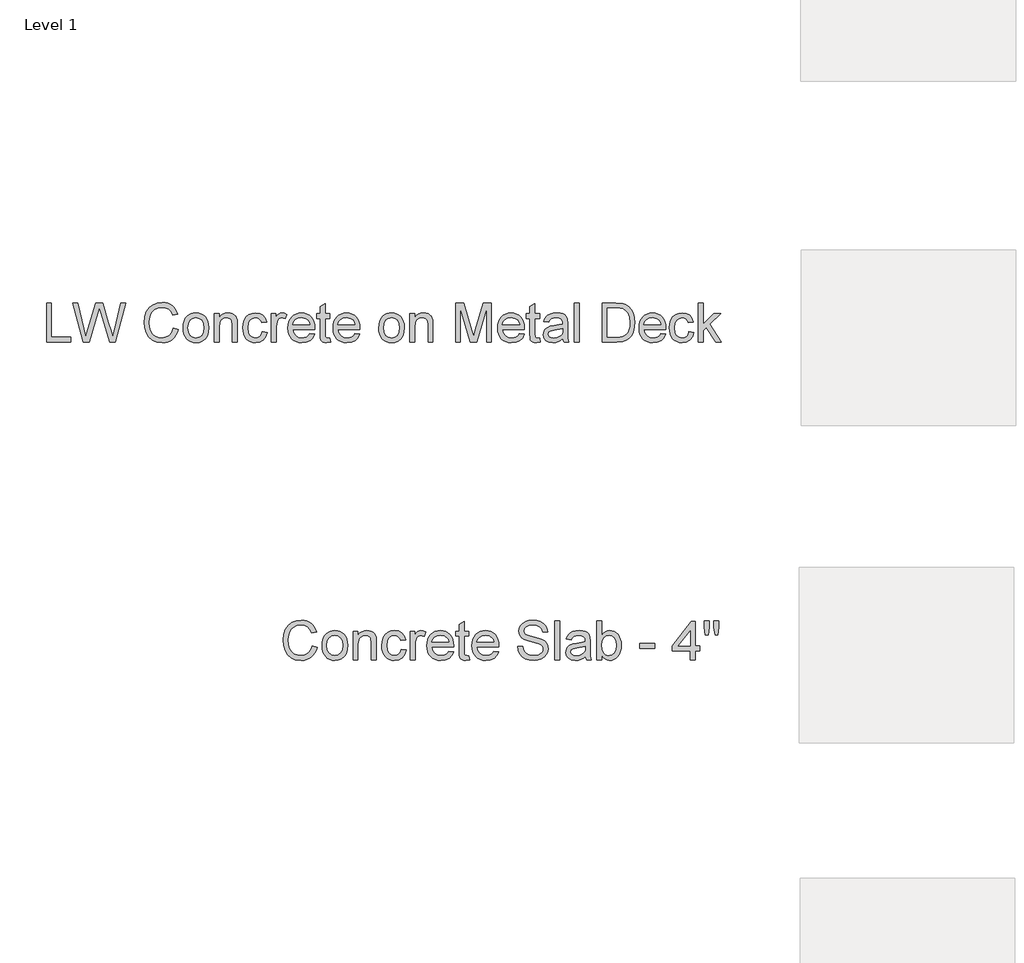
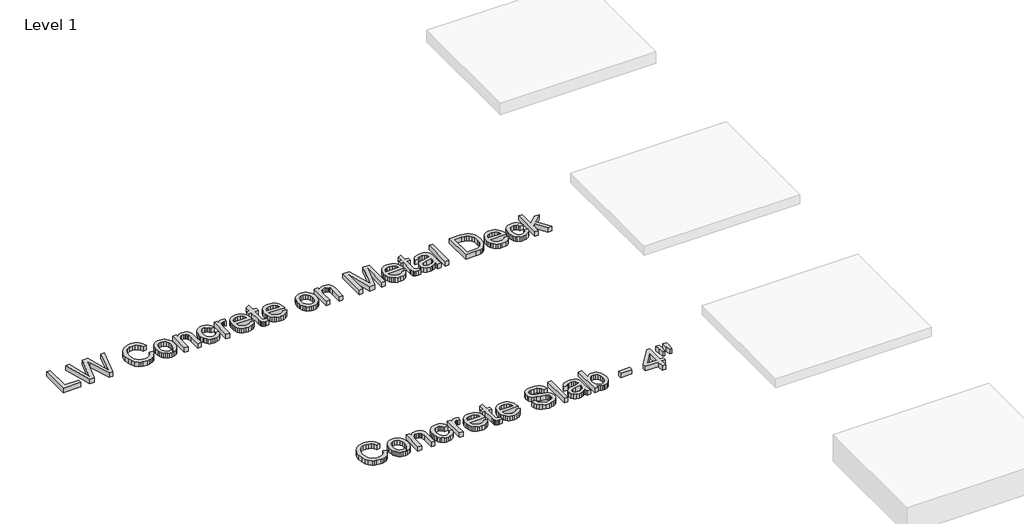
# One storey, part 13 of 42: 2 proxies.
"""IFC4 building model written with IfcOpenShell, lengths in millimetres."""

from ifc_helpers import new_model, si_unit, origin, origin_with_axes, place, context, project, spatial, polyline, outline, extrude, element, save

model = new_model("IFC4")

# Units and contexts
model_context = context("Model", 3, world=origin())
ifc_project = project(units=[si_unit("LENGTHUNIT", "METRE", prefix="MILLI")], contexts=[model_context])

# Site, building, storey
site = spatial("IfcSite", under=ifc_project)
building = spatial("IfcBuilding", under=site)
storey = spatial("IfcBuildingStorey", under=building, Name="Level 1", Elevation=0.0)

# Proxies
placement = place(None, origin())
element("IfcBuildingElementProxy", 1, Name="8\" Arial", ObjectType="8\" Arial", at=placement, inside=storey, context=model_context, shape_type="SweptSolid", body=[
    extrude(outline(polyline([(17896.3774302, -8659.233143), (17896.3774302, -8354.6660489), (17934.448317, -8354.6660489), (17934.448317, -8621.1622562), (18086.731864, -8621.1622562), (18086.731864, -8659.233143), (17896.3774302, -8659.233143)])), origin_with_axes(), (0.0, 0.0, 1.0), 50.8),
    extrude(outline(polyline([(18184.0654397, -8659.233143), (18101.0084465, -8354.6660489), (18140.2690485, -8354.6660489), (18188.4525146, -8554.8356332), (18203.3239547, -8616.626467), (18219.2363956, -8561.9739245), (18279.6144426, -8354.6660489), (18336.2002723, -8354.6660489), (18380.0710208, -8504.9419515), (18398.8648032, -8560.7098521), (18412.7138319, -8616.626467), (18427.1391288, -8556.620206), (18475.7687381, -8354.6660489), (18515.02934, -8354.6660489), (18431.8979897, -8659.233143), (18391.2246009, -8659.233143), (18318.2058298, -8424.2643888), (18308.0188933, -8391.4728633), (18296.5678844, -8430.9565368), (18230.0181897, -8659.233143), (18184.0654397, -8659.233143)])), origin_with_axes(), (0.0, 0.0, 1.0), 50.8),
    extrude(outline(polyline([(18886.2204859, -8550.9690588), (18924.2913727, -8560.7842093), (18916.7580588, -8584.4600067), (18906.724484, -8605.1475741), (18894.1906484, -8622.8469116), (18879.1565519, -8637.558019), (18861.9614492, -8649.1228874), (18842.9445951, -8657.3835076), (18822.1059896, -8662.3398798), (18799.4456327, -8663.9920038), (18755.2867501, -8658.9914821), (18736.6161218, -8652.7408299), (18720.2180354, -8643.9899168), (18693.3379073, -8619.5078085), (18673.7447849, -8586.0656575), (18661.7825703, -8546.7492876), (18657.7951654, -8504.6445227), (18662.3030707, -8460.2346846), (18675.8267865, -8421.8849584), (18697.6599196, -8390.8129431), (18727.0960764, -8368.236238), (18762.0067822, -8354.4894506), (18800.2635619, -8349.9071881), (18822.0386034, -8351.3896848), (18842.0058355, -8355.8371748), (18860.1652581, -8363.2496583), (18876.5168712, -8373.6271351), (18890.7911301, -8386.6954131), (18902.7184898, -8402.1803002), (18919.5325118, -8440.3999013), (18881.4616251, -8449.4714798), (18868.263222, -8421.70836), (18850.2316008, -8402.663622), (18827.14369, -8391.6494616), (18798.7764179, -8387.9780748), (18766.0778389, -8392.0491316), (18739.2163001, -8404.2623018), (18718.8331325, -8423.3349238), (18705.5696668, -8447.9843358), (18698.2919558, -8475.8496968), (18695.8660521, -8504.5701655), (18698.738099, -8539.7411215), (18707.3542396, -8570.1532165), (18722.0397868, -8594.6446195), (18743.1200532, -8612.0534991), (18768.3922068, -8622.4542126), (18795.6534155, -8625.9211171), (18827.4318241, -8621.1994348), (18853.9122822, -8607.0343881), (18873.9050746, -8583.5746913), (18886.2204859, -8550.9690588)])), origin_with_axes(), (0.0, 0.0, 1.0), 50.8),
    extrude(outline(polyline([(18962.3622594, -8547.3999131), (18964.4210244, -8518.4331361), (18970.5973194, -8493.4723533), (18980.8911444, -8472.5175647), (18995.3024994, -8455.5687703), (19009.8114481, -8444.7358556), (19025.8261302, -8436.9980594), (19043.3465457, -8432.3553817), (19062.3726944, -8430.8078224), (19083.3762799, -8432.6923127), (19102.3675737, -8438.3457837), (19119.3465758, -8447.7682352), (19134.3132861, -8460.9596673), (19146.5287799, -8477.4739369), (19155.2541327, -8496.8649006), (19160.4893444, -8519.1325586), (19162.2344149, -8544.2769107), (19159.1485911, -8582.7381728), (19149.8911196, -8612.0163205), (19134.7315453, -8633.9424001), (19113.9394131, -8650.3474575), (19089.2435278, -8660.5808673), (19062.3726944, -8663.9920038), (19041.0623854, -8662.1144845), (19021.8944933, -8656.4819266), (19004.869018, -8647.09433), (18989.9859595, -8633.9516947), (18977.9005907, -8617.2770925), (18969.2681845, -8597.2935948), (18964.0887407, -8574.0012017), (18962.3622594, -8547.3999131)]), holes=[polyline([(19000.4331462, -8547.3255559), (19004.8388103, -8581.7808238), (19018.0558028, -8606.3279947), (19037.946354, -8621.0228365), (19062.3726944, -8625.9211171), (19086.687499, -8620.9949525), (19106.5408716, -8606.2164589), (19119.757864, -8581.3439753), (19124.1635282, -8546.1358407), (19119.7299801, -8512.6843951), (19106.4293358, -8488.4718316), (19086.5480793, -8473.7769898), (19062.3726944, -8468.8787092), (19037.946354, -8473.7584005), (19018.0558028, -8488.3974744), (19004.8388103, -8512.8888774), (19000.4331462, -8547.3255559)])]), origin_with_axes(), (0.0, 0.0, 1.0), 50.8),
    extrude(outline(polyline([(19205.0641625, -8659.233143), (19205.0641625, -8435.5666833), (19243.1350493, -8435.5666833), (19243.1350493, -8466.7967076), (19256.3613364, -8451.0515703), (19272.2458934, -8439.8050437), (19290.7887203, -8433.0571278), (19311.9898171, -8430.8078224), (19330.7557157, -8432.6202792), (19347.9415237, -8438.0576495), (19362.2738741, -8446.4414239), (19372.4793999, -8457.0930929), (19383.8932302, -8485.0885789), (19385.9008746, -8521.8953933), (19385.9008746, -8659.233143), (19347.8299879, -8659.233143), (19347.8299879, -8527.0260401), (19343.442913, -8493.3422282), (19337.3735065, -8483.3133008), (19327.9394367, -8475.5336787), (19315.8470969, -8470.5424516), (19301.8028806, -8468.8787092), (19279.5050151, -8472.6151585), (19260.4974557, -8483.8245065), (19252.9014029, -8492.9750895), (19247.4756509, -8505.4810412), (19243.1350493, -8540.5590507), (19243.1350493, -8659.233143), (19205.0641625, -8659.233143)])), origin_with_axes(), (0.0, 0.0, 1.0), 50.8),
    extrude(outline(polyline([(19581.0141693, -8578.3325086), (19619.085056, -8583.0913695), (19608.4705656, -8616.9517797), (19588.5242465, -8642.5399514), (19561.1236181, -8658.6289907), (19528.1461996, -8663.9920038), (19506.7940647, -8662.1214555), (19487.6494091, -8656.5098105), (19470.712233, -8647.1570689), (19455.9825363, -8634.0632306), (19444.0598239, -8617.4746038), (19435.5436008, -8597.6374969), (19430.4338669, -8574.5519097), (19428.7306222, -8548.2178423), (19431.6398477, -8514.3388428), (19440.3675241, -8484.9770431), (19455.0530713, -8461.2663908), (19475.8359089, -8444.340833), (19500.6990979, -8434.1910751), (19527.6256992, -8430.8078224), (19559.7944831, -8435.4551475), (19585.5127799, -8449.3971226), (19603.9626603, -8471.8901758), (19614.3261952, -8502.1907351), (19576.2553084, -8506.949596), (19569.3493834, -8490.3400562), (19558.5954733, -8478.4336095), (19544.5884356, -8471.2674343), (19527.923128, -8468.8787092), (19503.3201892, -8473.5818021), (19483.7921294, -8487.691081), (19471.0491641, -8511.968707), (19466.801509, -8547.1768415), (19470.9562176, -8582.8590032), (19483.4203434, -8607.2202811), (19502.5952065, -8621.2459081), (19526.8821272, -8625.9211171), (19546.59608, -8623.0025969), (19562.7594765, -8614.2470366), (19574.5172089, -8599.4313643), (19581.0141693, -8578.3325086)])), origin_with_axes(), (0.0, 0.0, 1.0), 50.8),
    extrude(outline(polyline([(19652.3970819, -8659.233143), (19652.3970819, -8435.5666833), (19685.7091079, -8435.5666833), (19685.7091079, -8468.6556376), (19698.0152246, -8449.4714798), (19709.3546977, -8438.1691853), (19720.7313494, -8432.6481632), (19733.1490019, -8430.8078224), (19752.1100881, -8433.7449319), (19771.3686031, -8442.5562601), (19758.6535217, -8476.6862153), (19745.2692256, -8470.8305857), (19731.8849295, -8468.8787092), (19720.5175724, -8470.7562285), (19710.3585199, -8476.3887865), (19702.1513439, -8485.3488291), (19696.6396164, -8497.2088027), (19692.0108806, -8518.4749621), (19690.4679687, -8541.6744087), (19690.4679687, -8659.233143), (19652.3970819, -8659.233143)])), origin_with_axes(), (0.0, 0.0, 1.0), 50.8),
    extrude(outline(polyline([(19951.759172, -8592.6090912), (19989.0864867, -8597.367952), (19975.637128, -8625.4935632), (19954.175781, -8646.5180617), (19925.1857674, -8659.6235183), (19889.150409, -8663.9920038), (19865.5280558, -8662.1075135), (19844.4803207, -8656.4540426), (19826.0072036, -8647.0315911), (19810.1087046, -8633.8401589), (19797.3239134, -8617.2468849), (19788.1919197, -8597.6189076), (19782.7127235, -8574.956227), (19780.8863248, -8549.2588432), (19782.7313128, -8522.6900859), (19788.2662769, -8499.272215), (19797.4912171, -8479.0052305), (19810.4061334, -8461.8891323), (19826.2628065, -8448.2910593), (19844.313017, -8438.5781499), (19864.5567648, -8432.7504043), (19886.9940502, -8430.8078224), (19908.7086764, -8432.745757), (19928.3459484, -8438.5595606), (19945.9058661, -8448.2492333), (19961.3884295, -8461.8147751), (19974.0268299, -8478.8936947), (19983.0542588, -8499.1235006), (19988.4707161, -8522.5041929), (19990.2762019, -8549.0357715), (19990.0531303, -8559.2970652), (19818.9572115, -8559.2970652), (19825.5471184, -8587.7944624), (19840.8554071, -8608.7446037), (19862.9487904, -8621.6269887), (19889.893981, -8625.9211171), (19910.1563182, -8623.932062), (19927.2212957, -8617.9648966), (19941.0889137, -8607.647835), (19951.759172, -8592.6090912)]), holes=[polyline([(19818.9572115, -8521.2261785), (19952.2053152, -8521.2261785), (19947.056079, -8501.1125557), (19936.962089, -8486.7244374), (19914.7664646, -8473.3401412), (19886.8453358, -8468.8787092), (19861.1828069, -8472.4385602), (19839.9631207, -8483.1181131), (19825.212511, -8499.7648314), (19818.9572115, -8521.2261785)])]), origin_with_axes(), (0.0, 0.0, 1.0), 50.8),
    extrude(outline(polyline([(20109.247723, -8627.4826183), (20114.0065839, -8660.348501), (20085.527776, -8663.9920038), (20067.254494, -8662.4119133), (20053.6285369, -8657.6716418), (20043.9992794, -8650.3660468), (20037.716096, -8641.089986), (20034.2584861, -8625.1589558), (20033.1059495, -8597.8884524), (20033.1059495, -8473.63757), (20004.5527845, -8473.63757), (20004.5527845, -8435.5666833), (20033.1059495, -8435.5666833), (20033.1059495, -8381.2115696), (20071.1768363, -8358.8300522), (20071.1768363, -8435.5666833), (20109.247723, -8435.5666833), (20109.247723, -8473.63757), (20071.1768363, -8473.63757), (20071.1768363, -8596.7730944), (20073.1844807, -8616.4033954), (20079.6907358, -8623.3557936), (20092.6660673, -8625.9211171), (20109.247723, -8627.4826183)])), origin_with_axes(), (0.0, 0.0, 1.0), 50.8),
    extrude(outline(polyline([(20303.9148745, -8592.6090912), (20341.2421892, -8597.367952), (20327.7928306, -8625.4935632), (20306.3314835, -8646.5180617), (20277.3414699, -8659.6235183), (20241.3061115, -8663.9920038), (20217.6837583, -8662.1075135), (20196.6360232, -8656.4540426), (20178.1629061, -8647.0315911), (20162.2644071, -8633.8401589), (20149.479616, -8617.2468849), (20140.3476222, -8597.6189076), (20134.868426, -8574.956227), (20133.0420273, -8549.2588432), (20134.8870153, -8522.6900859), (20140.4219794, -8499.272215), (20149.6469197, -8479.0052305), (20162.5618359, -8461.8891323), (20178.418509, -8448.2910593), (20196.4687195, -8438.5781499), (20216.7124674, -8432.7504043), (20239.1497527, -8430.8078224), (20260.8643789, -8432.745757), (20280.5016509, -8438.5595606), (20298.0615686, -8448.2492333), (20313.544132, -8461.8147751), (20326.1825324, -8478.8936947), (20335.2099613, -8499.1235006), (20340.6264187, -8522.5041929), (20342.4319044, -8549.0357715), (20342.2088328, -8559.2970652), (20171.112914, -8559.2970652), (20177.7028209, -8587.7944624), (20193.0111096, -8608.7446037), (20215.1044929, -8621.6269887), (20242.0496835, -8625.9211171), (20262.3120207, -8623.932062), (20279.3769982, -8617.9648966), (20293.2446162, -8607.647835), (20303.9148745, -8592.6090912)]), holes=[polyline([(20171.112914, -8521.2261785), (20304.3610177, -8521.2261785), (20299.2117815, -8501.1125557), (20289.1177915, -8486.7244374), (20266.9221671, -8473.3401412), (20239.0010383, -8468.8787092), (20213.3385094, -8472.4385602), (20192.1188232, -8483.1181131), (20177.3682135, -8499.7648314), (20171.112914, -8521.2261785)])]), origin_with_axes(), (0.0, 0.0, 1.0), 50.8),
    extrude(outline(polyline([(20489.9565906, -8547.3999131), (20492.0153556, -8518.4331361), (20498.1916506, -8493.4723533), (20508.4854756, -8472.5175647), (20522.8968305, -8455.5687703), (20537.4057793, -8444.7358556), (20553.4204614, -8436.9980594), (20570.9408768, -8432.3553817), (20589.9670256, -8430.8078224), (20610.9706111, -8432.6923127), (20629.9619049, -8438.3457837), (20646.9409069, -8447.7682352), (20661.9076173, -8460.9596673), (20674.1231111, -8477.4739369), (20682.8484639, -8496.8649006), (20688.0836756, -8519.1325586), (20689.8287461, -8544.2769107), (20686.7429223, -8582.7381728), (20677.4854508, -8612.0163205), (20662.3258765, -8633.9424001), (20641.5337443, -8650.3474575), (20616.837859, -8660.5808673), (20589.9670256, -8663.9920038), (20568.6567166, -8662.1144845), (20549.4888244, -8656.4819266), (20532.4633491, -8647.09433), (20517.5802907, -8633.9516947), (20505.4949219, -8617.2770925), (20496.8625156, -8597.2935948), (20491.6830719, -8574.0012017), (20489.9565906, -8547.3999131)]), holes=[polyline([(20528.0274774, -8547.3255559), (20532.4331415, -8581.7808238), (20545.650134, -8606.3279947), (20565.5406851, -8621.0228365), (20589.9670256, -8625.9211171), (20614.2818302, -8620.9949525), (20634.1352028, -8606.2164589), (20647.3521952, -8581.3439753), (20651.7578594, -8546.1358407), (20647.3243113, -8512.6843951), (20634.023667, -8488.4718316), (20614.1424105, -8473.7769898), (20589.9670256, -8468.8787092), (20565.5406851, -8473.7584005), (20545.650134, -8488.3974744), (20532.4331415, -8512.8888774), (20528.0274774, -8547.3255559)])]), origin_with_axes(), (0.0, 0.0, 1.0), 50.8),
    extrude(outline(polyline([(20732.6584937, -8659.233143), (20732.6584937, -8435.5666833), (20770.7293805, -8435.5666833), (20770.7293805, -8466.7967076), (20783.9556676, -8451.0515703), (20799.8402246, -8439.8050437), (20818.3830515, -8433.0571278), (20839.5841483, -8430.8078224), (20858.3500469, -8432.6202792), (20875.5358549, -8438.0576495), (20889.8682053, -8446.4414239), (20900.0737311, -8457.0930929), (20911.4875614, -8485.0885789), (20913.4952058, -8521.8953933), (20913.4952058, -8659.233143), (20875.4243191, -8659.233143), (20875.4243191, -8527.0260401), (20871.0372442, -8493.3422282), (20864.9678377, -8483.3133008), (20855.5337679, -8475.5336787), (20843.4414281, -8470.5424516), (20829.3972118, -8468.8787092), (20807.0993463, -8472.6151585), (20788.0917868, -8483.8245065), (20780.4957341, -8492.9750895), (20775.0699821, -8505.4810412), (20770.7293805, -8540.5590507), (20770.7293805, -8659.233143), (20732.6584937, -8659.233143)])), origin_with_axes(), (0.0, 0.0, 1.0), 50.8),
    extrude(outline(polyline([(21089.5730571, -8659.233143), (21089.5730571, -8354.6660489), (21155.0817509, -8354.6660489), (21217.3930851, -8569.3352873), (21229.959452, -8614.1726794), (21243.5668197, -8565.6174273), (21304.8371531, -8354.6660489), (21370.3458469, -8354.6660489), (21370.3458469, -8659.233143), (21332.2749602, -8659.233143), (21332.2749602, -8392.7369357), (21255.7614006, -8659.233143), (21204.1575034, -8659.233143), (21127.6439438, -8392.7369357), (21127.6439438, -8659.233143), (21089.5730571, -8659.233143)])), origin_with_axes(), (0.0, 0.0, 1.0), 50.8),
    extrude(outline(polyline([(21588.8073026, -8592.6090912), (21626.1346173, -8597.367952), (21612.6852587, -8625.4935632), (21591.2239116, -8646.5180617), (21562.233898, -8659.6235183), (21526.1985396, -8663.9920038), (21502.5761864, -8662.1075135), (21481.5284513, -8656.4540426), (21463.0553342, -8647.0315911), (21447.1568352, -8633.8401589), (21434.3720441, -8617.2468849), (21425.2400503, -8597.6189076), (21419.7608541, -8574.956227), (21417.9344554, -8549.2588432), (21419.7794434, -8522.6900859), (21425.3144075, -8499.272215), (21434.5393478, -8479.0052305), (21447.454264, -8461.8891323), (21463.3109371, -8448.2910593), (21481.3611476, -8438.5781499), (21501.6048955, -8432.7504043), (21524.0421808, -8430.8078224), (21545.756807, -8432.745757), (21565.394079, -8438.5595606), (21582.9539967, -8448.2492333), (21598.4365601, -8461.8147751), (21611.0749605, -8478.8936947), (21620.1023894, -8499.1235006), (21625.5188468, -8522.5041929), (21627.3243325, -8549.0357715), (21627.1012609, -8559.2970652), (21456.0053421, -8559.2970652), (21462.595249, -8587.7944624), (21477.9035377, -8608.7446037), (21499.996921, -8621.6269887), (21526.9421116, -8625.9211171), (21547.2044488, -8623.932062), (21564.2694264, -8617.9648966), (21578.1370443, -8607.647835), (21588.8073026, -8592.6090912)]), holes=[polyline([(21456.0053421, -8521.2261785), (21589.2534458, -8521.2261785), (21584.1042096, -8501.1125557), (21574.0102196, -8486.7244374), (21551.8145952, -8473.3401412), (21523.8934664, -8468.8787092), (21498.2309375, -8472.4385602), (21477.0112513, -8483.1181131), (21462.2606416, -8499.7648314), (21456.0053421, -8521.2261785)])]), origin_with_axes(), (0.0, 0.0, 1.0), 50.8),
    extrude(outline(polyline([(21746.2958537, -8627.4826183), (21751.0547145, -8660.348501), (21722.5759066, -8663.9920038), (21704.3026246, -8662.4119133), (21690.6766675, -8657.6716418), (21681.04741, -8650.3660468), (21674.7642266, -8641.089986), (21671.3066168, -8625.1589558), (21670.1540801, -8597.8884524), (21670.1540801, -8473.63757), (21641.6009151, -8473.63757), (21641.6009151, -8435.5666833), (21670.1540801, -8435.5666833), (21670.1540801, -8381.2115696), (21708.2249669, -8358.8300522), (21708.2249669, -8435.5666833), (21746.2958537, -8435.5666833), (21746.2958537, -8473.63757), (21708.2249669, -8473.63757), (21708.2249669, -8596.7730944), (21710.2326113, -8616.4033954), (21716.7388664, -8623.3557936), (21729.7141979, -8625.9211171), (21746.2958537, -8627.4826183)])), origin_with_axes(), (0.0, 0.0, 1.0), 50.8),
    extrude(outline(polyline([(21927.1325658, -8630.6799779), (21908.9429355, -8646.2764008), (21890.2142156, -8656.4819266), (21870.5188521, -8662.1144845), (21849.429291, -8663.9920038), (21817.6137038, -8659.4748039), (21794.1447123, -8645.9232041), (21779.6729421, -8625.3448488), (21774.8490187, -8599.7473824), (21776.6707702, -8583.9650666), (21782.1360244, -8569.6327161), (21790.566272, -8557.363778), (21801.2830036, -8547.7716991), (21827.94006, -8535.2796894), (21860.8802999, -8529.554185), (21899.8062945, -8523.5312517), (21926.9094942, -8516.4673176), (21927.1325658, -8507.9905968), (21924.5114744, -8490.9999764), (21916.6482005, -8479.8835749), (21899.0627225, -8471.6299256), (21874.5620249, -8468.8787092), (21851.8830787, -8470.7097553), (21836.0449949, -8476.2028935), (21825.2446115, -8486.361946), (21817.6787663, -8502.1907351), (21779.6078796, -8497.4318743), (21786.2163758, -8476.6118581), (21796.0779995, -8460.2532739), (21810.1129212, -8447.7426749), (21829.241311, -8438.4666141), (21852.6359453, -8432.7225204), (21879.4696001, -8430.8078224), (21905.2064862, -8432.4994488), (21925.6082432, -8437.5743277), (21940.990889, -8445.2052354), (21951.670442, -8454.5649481), (21958.7529654, -8466.1367874), (21963.3445225, -8480.4040753), (21965.2034525, -8513.7161012), (21965.2034525, -8561.0816381), (21967.1367397, -8627.2223681), (21974.7211742, -8659.233143), (21936.6502875, -8659.233143), (21930.552997, -8645.9975613), (21927.1325658, -8630.6799779)]), holes=[polyline([(21927.1325658, -8554.5382044), (21865.713518, -8566.2122849), (21832.9591711, -8572.3839326), (21818.1249095, -8582.4221547), (21812.9199055, -8597.0705232), (21815.7547738, -8608.391407), (21824.2593786, -8617.6674678), (21838.247827, -8623.8577048), (21857.5342259, -8625.9211171), (21877.9824561, -8623.6439278), (21896.0512559, -8616.81236), (21910.6996244, -8606.7462539), (21920.8865609, -8594.76545), (21925.4037609, -8582.4221547), (21926.9094942, -8565.3199985), (21927.1325658, -8554.5382044)])]), origin_with_axes(), (0.0, 0.0, 1.0), 50.8),
    extrude(outline(polyline([(22017.5509218, -8659.233143), (22017.5509218, -8354.6660489), (22055.6218086, -8354.6660489), (22055.6218086, -8659.233143), (22017.5509218, -8659.233143)])), origin_with_axes(), (0.0, 0.0, 1.0), 50.8),
    extrude(outline(polyline([(22236.4585207, -8659.233143), (22236.4585207, -8354.6660489), (22341.5252453, -8354.6660489), (22395.880359, -8359.0531238), (22420.157985, -8367.5112553), (22440.6433938, -8380.8397836), (22461.7050709, -8404.0392302), (22476.7066361, -8432.8898241), (22485.6852681, -8466.8338862), (22488.6781455, -8505.3137375), (22486.6519117, -8538.0030219), (22480.5732106, -8566.7699639), (22471.3157391, -8591.2613669), (22459.7531944, -8611.1240341), (22446.4432555, -8626.8041088), (22431.9436013, -8638.7477342), (22415.296883, -8647.6055357), (22395.5457516, -8654.0281389), (22346.5815349, -8659.233143), (22236.4585207, -8659.233143)]), holes=[polyline([(22274.5294074, -8621.1622562), (22341.8970313, -8621.1622562), (22369.7623922, -8619.786648), (22390.8984265, -8615.6598234), (22406.8480461, -8609.0234432), (22419.1541628, -8600.1191684), (22432.3804499, -8583.6397538), (22442.3164308, -8562.3085319), (22448.5345517, -8536.0325561), (22450.6072587, -8504.7188799), (22446.5454966, -8463.2275619), (22434.3602103, -8432.5923953), (22416.3564731, -8411.5493075), (22394.8393582, -8398.8342261), (22372.9411626, -8394.2612583), (22340.8560305, -8392.7369357), (22274.5294074, -8392.7369357), (22274.5294074, -8621.1622562)])]), origin_with_axes(), (0.0, 0.0, 1.0), 50.8),
    extrude(outline(polyline([(22692.8630186, -8592.6090912), (22730.1903333, -8597.367952), (22716.7409747, -8625.4935632), (22695.2796276, -8646.5180617), (22666.289614, -8659.6235183), (22630.2542556, -8663.9920038), (22606.6319024, -8662.1075135), (22585.5841673, -8656.4540426), (22567.1110502, -8647.0315911), (22551.2125512, -8633.8401589), (22538.42776, -8617.2468849), (22529.2957663, -8597.6189076), (22523.8165701, -8574.956227), (22521.9901714, -8549.2588432), (22523.8351594, -8522.6900859), (22529.3701235, -8499.272215), (22538.5950638, -8479.0052305), (22551.50998, -8461.8891323), (22567.3666531, -8448.2910593), (22585.4168636, -8438.5781499), (22605.6606115, -8432.7504043), (22628.0978968, -8430.8078224), (22649.812523, -8432.745757), (22669.449795, -8438.5595606), (22687.0097127, -8448.2492333), (22702.4922761, -8461.8147751), (22715.1306765, -8478.8936947), (22724.1581054, -8499.1235006), (22729.5745628, -8522.5041929), (22731.3800485, -8549.0357715), (22731.1569769, -8559.2970652), (22560.0610581, -8559.2970652), (22566.650965, -8587.7944624), (22581.9592537, -8608.7446037), (22604.052637, -8621.6269887), (22630.9978276, -8625.9211171), (22651.2601648, -8623.932062), (22668.3251423, -8617.9648966), (22682.1927603, -8607.647835), (22692.8630186, -8592.6090912)]), holes=[polyline([(22560.0610581, -8521.2261785), (22693.3091618, -8521.2261785), (22688.1599256, -8501.1125557), (22678.0659356, -8486.7244374), (22655.8703112, -8473.3401412), (22627.9491824, -8468.8787092), (22602.2866535, -8472.4385602), (22581.0669673, -8483.1181131), (22566.3163576, -8499.7648314), (22560.0610581, -8521.2261785)])]), origin_with_axes(), (0.0, 0.0, 1.0), 50.8),
    extrude(outline(polyline([(22912.2167606, -8578.3325086), (22950.2876474, -8583.0913695), (22939.673157, -8616.9517797), (22919.7268379, -8642.5399514), (22892.3262095, -8658.6289907), (22859.3487909, -8663.9920038), (22837.996656, -8662.1214555), (22818.8520005, -8656.5098105), (22801.9148244, -8647.1570689), (22787.1851277, -8634.0632306), (22775.2624153, -8617.4746038), (22766.7461921, -8597.6374969), (22761.6364582, -8574.5519097), (22759.9332136, -8548.2178423), (22762.8424391, -8514.3388428), (22771.5701155, -8484.9770431), (22786.2556627, -8461.2663908), (22807.0385003, -8444.340833), (22831.9016892, -8434.1910751), (22858.8282905, -8430.8078224), (22890.9970745, -8435.4551475), (22916.7153713, -8449.3971226), (22935.1652517, -8471.8901758), (22945.5287866, -8502.1907351), (22907.4578998, -8506.949596), (22900.5519748, -8490.3400562), (22889.7980646, -8478.4336095), (22875.791027, -8471.2674343), (22859.1257193, -8468.8787092), (22834.5227806, -8473.5818021), (22814.9947207, -8487.691081), (22802.2517555, -8511.968707), (22798.0041004, -8547.1768415), (22802.158809, -8582.8590032), (22814.6229347, -8607.2202811), (22833.7977979, -8621.2459081), (22858.0847185, -8625.9211171), (22877.7986714, -8623.0025969), (22893.9620679, -8614.2470366), (22905.7198002, -8599.4313643), (22912.2167606, -8578.3325086)])), origin_with_axes(), (0.0, 0.0, 1.0), 50.8),
    extrude(outline(polyline([(22983.5996733, -8659.233143), (22983.5996733, -8354.6660489), (23021.6705601, -8354.6660489), (23021.6705601, -8518.3262477), (23107.0326265, -8435.5666833), (23159.6775246, -8435.5666833), (23073.2744574, -8519.3672485), (23164.4363854, -8659.233143), (23119.9707794, -8659.233143), (23045.9853647, -8545.8384119), (23021.6705601, -8569.4096445), (23021.6705601, -8659.233143), (22983.5996733, -8659.233143)])), origin_with_axes(), (0.0, 0.0, 1.0), 50.8),
])
element("IfcBuildingElementProxy", 2, Name="8\" Arial", ObjectType="8\" Arial", at=placement, inside=storey, context=model_context, shape_type="SweptSolid", body=[
    extrude(outline(polyline([(19971.0152117, -11032.4410941), (20009.0860985, -11042.2562446), (20001.5527846, -11065.932042), (19991.5192098, -11086.6196095), (19978.9853741, -11104.3189469), (19963.9512776, -11119.0300543), (19946.756175, -11130.5949227), (19927.7393209, -11138.855543), (19906.9007154, -11143.8119151), (19884.2403585, -11145.4640392), (19840.0814759, -11140.4635174), (19821.4108475, -11134.2128652), (19805.0127611, -11125.4619522), (19778.1326331, -11100.9798438), (19758.5395107, -11067.5376928), (19746.577296, -11028.221323), (19742.5898911, -10986.1165581), (19747.0977964, -10941.7067199), (19760.6215123, -10903.3569937), (19782.4546454, -10872.2849784), (19811.8908022, -10849.7082734), (19846.8015079, -10835.9614859), (19885.0582877, -10831.3792234), (19906.8333292, -10832.8617201), (19926.8005612, -10837.3092102), (19944.9599838, -10844.7216936), (19961.311597, -10855.0991704), (19975.5858559, -10868.1674485), (19987.5132156, -10883.6523355), (20004.3272376, -10921.8719367), (19966.2563508, -10930.9435151), (19953.0579477, -10903.1803953), (19935.0263266, -10884.1356573), (19911.9384157, -10873.1214969), (19883.5711437, -10869.4501102), (19850.8725647, -10873.5211669), (19824.0110259, -10885.7343371), (19803.6278583, -10904.8069591), (19790.3643926, -10929.4563711), (19783.0866816, -10957.3217321), (19780.6607779, -10986.0422009), (19783.5328248, -11021.2131568), (19792.1489654, -11051.6252519), (19806.8345125, -11076.1166549), (19827.9147789, -11093.5255345), (19853.1869325, -11103.9262479), (19880.4481412, -11107.3931524), (19912.2265499, -11102.6714702), (19938.707008, -11088.5064234), (19958.6998003, -11065.0467266), (19971.0152117, -11032.4410941)])), origin_with_axes(), (0.0, 0.0, 1.0), 50.8),
    extrude(outline(polyline([(20047.1569852, -11028.8719485), (20049.2157502, -10999.9051715), (20055.3920452, -10974.9443887), (20065.6858702, -10953.9896), (20080.0972251, -10937.0408056), (20094.6061739, -10926.2078909), (20110.620856, -10918.4700947), (20128.1412714, -10913.827417), (20147.1674202, -10912.2798578), (20168.1710057, -10914.1643481), (20187.1622995, -10919.817819), (20204.1413015, -10929.2402705), (20219.1080118, -10942.4317027), (20231.3235057, -10958.9459722), (20240.0488585, -10978.3369359), (20245.2840701, -11000.6045939), (20247.0291407, -11025.748946), (20243.9433169, -11064.2102081), (20234.6858454, -11093.4883559), (20219.5262711, -11115.4144354), (20198.7341388, -11131.8194928), (20174.0382536, -11142.0529026), (20147.1674202, -11145.4640392), (20125.8571112, -11143.5865198), (20106.689219, -11137.9539619), (20089.6637437, -11128.5663653), (20074.7806853, -11115.4237301), (20062.6953165, -11098.7491278), (20054.0629102, -11078.7656301), (20048.8834665, -11055.473237), (20047.1569852, -11028.8719485)]), holes=[polyline([(20085.227872, -11028.7975913), (20089.6335361, -11063.2528591), (20102.8505285, -11087.80003), (20122.7410797, -11102.4948718), (20147.1674202, -11107.3931524), (20171.4822248, -11102.4669879), (20191.3355974, -11087.6884942), (20204.5525898, -11062.8160106), (20208.9582539, -11027.6078761), (20204.5247058, -10994.1564304), (20191.2240616, -10969.9438669), (20171.342805, -10955.2490251), (20147.1674202, -10950.3507445), (20122.7410797, -10955.2304358), (20102.8505285, -10969.8695097), (20089.6335361, -10994.3609127), (20085.227872, -11028.7975913)])]), origin_with_axes(), (0.0, 0.0, 1.0), 50.8),
    extrude(outline(polyline([(20289.8588883, -11140.7051783), (20289.8588883, -10917.0387186), (20327.9297751, -10917.0387186), (20327.9297751, -10948.2687429), (20341.1560621, -10932.5236057), (20357.0406191, -10921.2770791), (20375.5834461, -10914.5291631), (20396.7845429, -10912.2798578), (20415.5504414, -10914.0923145), (20432.7362494, -10919.5296848), (20447.0685999, -10927.9134592), (20457.2741257, -10938.5651282), (20468.687956, -10966.5606143), (20470.6956004, -11003.3674286), (20470.6956004, -11140.7051783), (20432.6247136, -11140.7051783), (20432.6247136, -11008.4980755), (20428.2376388, -10974.8142636), (20422.1682323, -10964.7853361), (20412.7341625, -10957.005714), (20400.6418227, -10952.0144869), (20386.5976064, -10950.3507445), (20364.2997408, -10954.0871939), (20345.2921814, -10965.2965419), (20337.6961286, -10974.4471249), (20332.2703766, -10986.9530766), (20327.9297751, -11022.031086), (20327.9297751, -11140.7051783), (20289.8588883, -11140.7051783)])), origin_with_axes(), (0.0, 0.0, 1.0), 50.8),
    extrude(outline(polyline([(20665.808895, -11059.804544), (20703.8797818, -11064.5634048), (20693.2652914, -11098.4238151), (20673.3189723, -11124.0119868), (20645.9183439, -11140.1010261), (20612.9409253, -11145.4640392), (20591.5887904, -11143.5934908), (20572.4441349, -11137.9818458), (20555.5069588, -11128.6291042), (20540.7772621, -11115.5352659), (20528.8545497, -11098.9466391), (20520.3383265, -11079.1095322), (20515.2285926, -11056.023945), (20513.525348, -11029.6898777), (20516.4345735, -10995.8108781), (20525.1622499, -10966.4490785), (20539.8477971, -10942.7384261), (20560.6306346, -10925.8128683), (20585.4938236, -10915.6631104), (20612.4204249, -10912.2798578), (20644.5892089, -10916.9271828), (20670.3075057, -10930.8691579), (20688.7573861, -10953.3622112), (20699.120921, -10983.6627704), (20661.0500342, -10988.4216313), (20654.1441092, -10971.8120916), (20643.390199, -10959.9056448), (20629.3831613, -10952.7394696), (20612.7178537, -10950.3507445), (20588.114915, -10955.0538375), (20568.5868551, -10969.1631163), (20555.8438899, -10993.4407423), (20551.5962348, -11028.6488769), (20555.7509434, -11064.3310385), (20568.2150691, -11088.6923164), (20587.3899322, -11102.7179434), (20611.6768529, -11107.3931524), (20631.3908058, -11104.4746323), (20647.5542023, -11095.7190719), (20659.3119346, -11080.9033997), (20665.808895, -11059.804544)])), origin_with_axes(), (0.0, 0.0, 1.0), 50.8),
    extrude(outline(polyline([(20737.1918077, -11140.7051783), (20737.1918077, -10917.0387186), (20770.5038336, -10917.0387186), (20770.5038336, -10950.1276729), (20782.8099503, -10930.9435151), (20794.1494234, -10919.6412206), (20805.5260752, -10914.1201985), (20817.9437277, -10912.2798578), (20836.9048138, -10915.2169672), (20856.1633288, -10924.0282955), (20843.4482475, -10958.1582506), (20830.0639514, -10952.302621), (20816.6796553, -10950.3507445), (20805.3122982, -10952.2282638), (20795.1532457, -10957.8608218), (20786.9460696, -10966.8208645), (20781.4343421, -10978.680838), (20776.8056064, -10999.9469974), (20775.2626945, -11023.146444), (20775.2626945, -11140.7051783), (20737.1918077, -11140.7051783)])), origin_with_axes(), (0.0, 0.0, 1.0), 50.8),
    extrude(outline(polyline([(21036.5538977, -11074.0811265), (21073.8812125, -11078.8399873), (21060.4318538, -11106.9655985), (21038.9705068, -11127.990097), (21009.9804931, -11141.0955536), (20973.9451347, -11145.4640392), (20950.3227815, -11143.5795489), (20929.2750464, -11137.9260779), (20910.8019294, -11128.5036264), (20894.9034304, -11115.3121943), (20882.1186392, -11098.7189202), (20872.9866455, -11079.0909429), (20867.5074493, -11056.4282623), (20865.6810505, -11030.7308785), (20867.5260386, -11004.1621212), (20873.0610027, -10980.7442503), (20882.2859429, -10960.4772658), (20895.2008592, -10943.3611677), (20911.0575322, -10929.7630946), (20929.1077427, -10920.0501852), (20949.3514906, -10914.2224396), (20971.7887759, -10912.2798578), (20993.5034022, -10914.2177923), (21013.1406742, -10920.0315959), (21030.7005918, -10929.7212687), (21046.1831552, -10943.2868105), (21058.8215557, -10960.36573), (21067.8489846, -10980.5955359), (21073.2654419, -11003.9762282), (21075.0709277, -11030.5078069), (21074.8478561, -11040.7691006), (20903.7519373, -11040.7691006), (20910.3418442, -11069.2664977), (20925.6501329, -11090.216639), (20947.7435161, -11103.0990241), (20974.6887067, -11107.3931524), (20994.9510439, -11105.4040973), (21012.0160215, -11099.4369319), (21025.8836394, -11089.1198703), (21036.5538977, -11074.0811265)]), holes=[polyline([(20903.7519373, -11002.6982138), (21037.0000409, -11002.6982138), (21031.8508048, -10982.584591), (21021.7568148, -10968.1964727), (20999.5611904, -10954.8121766), (20971.6400615, -10950.3507445), (20945.9775326, -10953.9105955), (20924.7578465, -10964.5901485), (20910.0072368, -10981.2368668), (20903.7519373, -11002.6982138)])]), origin_with_axes(), (0.0, 0.0, 1.0), 50.8),
    extrude(outline(polyline([(21194.0424488, -11108.9546536), (21198.8013097, -11141.8205363), (21170.3225018, -11145.4640392), (21152.0492197, -11143.8839486), (21138.4232627, -11139.1436771), (21128.7940052, -11131.8380821), (21122.5108217, -11122.5620213), (21119.0532119, -11106.6309911), (21117.9006753, -11079.3604877), (21117.9006753, -10955.1096054), (21089.3475102, -10955.1096054), (21089.3475102, -10917.0387186), (21117.9006753, -10917.0387186), (21117.9006753, -10862.6836049), (21155.9715621, -10840.3020875), (21155.9715621, -10917.0387186), (21194.0424488, -10917.0387186), (21194.0424488, -10955.1096054), (21155.9715621, -10955.1096054), (21155.9715621, -11078.2451297), (21157.9792065, -11097.8754307), (21164.4854615, -11104.827829), (21177.4607931, -11107.3931524), (21194.0424488, -11108.9546536)])), origin_with_axes(), (0.0, 0.0, 1.0), 50.8),
    extrude(outline(polyline([(21388.7096002, -11074.0811265), (21426.036915, -11078.8399873), (21412.5875563, -11106.9655985), (21391.1262093, -11127.990097), (21362.1361956, -11141.0955536), (21326.1008373, -11145.4640392), (21302.4784841, -11143.5795489), (21281.4307489, -11137.9260779), (21262.9576319, -11128.5036264), (21247.0591329, -11115.3121943), (21234.2743417, -11098.7189202), (21225.142348, -11079.0909429), (21219.6631518, -11056.4282623), (21217.836753, -11030.7308785), (21219.6817411, -11004.1621212), (21225.2167052, -10980.7442503), (21234.4416454, -10960.4772658), (21247.3565617, -10943.3611677), (21263.2132348, -10929.7630946), (21281.2634452, -10920.0501852), (21301.5071931, -10914.2224396), (21323.9444784, -10912.2798578), (21345.6591047, -10914.2177923), (21365.2963767, -10920.0315959), (21382.8562944, -10929.7212687), (21398.3388577, -10943.2868105), (21410.9772582, -10960.36573), (21420.0046871, -10980.5955359), (21425.4211444, -11003.9762282), (21427.2266302, -11030.5078069), (21427.0035586, -11040.7691006), (21255.9076398, -11040.7691006), (21262.4975467, -11069.2664977), (21277.8058354, -11090.216639), (21299.8992187, -11103.0990241), (21326.8444093, -11107.3931524), (21347.1067465, -11105.4040973), (21364.171724, -11099.4369319), (21378.0393419, -11089.1198703), (21388.7096002, -11074.0811265)]), holes=[polyline([(21255.9076398, -11002.6982138), (21389.1557435, -11002.6982138), (21384.0065073, -10982.584591), (21373.9125173, -10968.1964727), (21351.7168929, -10954.8121766), (21323.795764, -10950.3507445), (21298.1332351, -10953.9105955), (21276.913549, -10964.5901485), (21262.1629393, -10981.2368668), (21255.9076398, -11002.6982138)])]), origin_with_axes(), (0.0, 0.0, 1.0), 50.8),
    extrude(outline(polyline([(21574.7513164, -11036.0102397), (21612.8222032, -11036.0102397), (21617.1906887, -11057.1369794), (21625.0911413, -11074.1183051), (21637.4158473, -11087.5955477), (21655.0570932, -11098.2100381), (21676.6206814, -11105.0973738), (21700.7124144, -11107.3931524), (21721.9228059, -11105.6550528), (21740.4935168, -11100.4407541), (21755.5415553, -11092.1871049), (21766.1839296, -11081.3309536), (21772.5135863, -11068.8668278), (21774.6234719, -11055.7892551), (21773.0433814, -11043.0462898), (21768.3031098, -11032.0321295), (21758.6738523, -11022.6352383), (21742.426804, -11014.7440803), (21686.9935109, -11000.2072476), (21650.6049558, -10990.5872848), (21627.3218573, -10981.4320544), (21608.3700658, -10968.6240266), (21594.9392964, -10953.101961), (21586.9366027, -10935.2004649), (21584.2690381, -10915.2541458), (21587.5686389, -10892.9562802), (21597.4674412, -10872.164148), (21613.7051949, -10854.5414914), (21636.0216498, -10841.7520529), (21662.8088313, -10833.9724308), (21692.4587651, -10831.3792234), (21724.5810758, -10834.0932612), (21752.6880977, -10842.2353747), (21775.7760085, -10855.6382601), (21792.8409861, -10874.1346138), (21803.6413695, -10896.5718991), (21807.9354978, -10921.7975795), (21769.864611, -10921.7975795), (21762.8750342, -10899.0814546), (21748.3010228, -10882.6856919), (21725.5291301, -10872.7590056), (21693.9459091, -10869.4501102), (21661.6191161, -10872.721827), (21639.442081, -10882.5369775), (21626.6154639, -10896.9808637), (21622.3399248, -10914.1387878), (21625.3699808, -10928.768567), (21634.4601486, -10940.535594), (21655.9493796, -10951.0571379), (21696.6227683, -10961.8017534), (21738.5974081, -10972.0072792), (21763.9903922, -10980.911554), (21785.6934001, -10994.723404), (21800.8343851, -11011.7697923), (21809.7293653, -11031.8648258), (21812.6943586, -11054.8226115), (21809.2832221, -11078.291603), (21799.0498123, -11100.3663969), (21782.4123887, -11119.3646617), (21759.7892103, -11133.6040657), (21732.5837695, -11142.4990458), (21702.1995584, -11145.4640392), (21664.9001276, -11142.2666795), (21634.1998984, -11132.6746006), (21609.745674, -11116.6506239), (21591.1842578, -11094.1575707), (21579.2685163, -11066.7569422), (21574.7513164, -11036.0102397)])), origin_with_axes(), (0.0, 0.0, 1.0), 50.8),
    extrude(outline(polyline([(21865.0418279, -11140.7051783), (21865.0418279, -10836.1380843), (21903.1127147, -10836.1380843), (21903.1127147, -11140.7051783), (21865.0418279, -11140.7051783)])), origin_with_axes(), (0.0, 0.0, 1.0), 50.8),
    extrude(outline(polyline([(22102.9848702, -11112.1520133), (22084.79524, -11127.7484361), (22066.06652, -11137.9539619), (22046.3711565, -11143.5865198), (22025.2815954, -11145.4640392), (21993.4660082, -11140.9468392), (21969.9970167, -11127.3952394), (21955.5252465, -11106.8168841), (21950.7013231, -11081.2194178), (21952.5230746, -11065.4371019), (21957.9883288, -11051.1047515), (21966.4185764, -11038.8358134), (21977.135308, -11029.2437345), (22003.7923644, -11016.7517248), (22036.7326043, -11011.0262203), (22075.6585989, -11005.003287), (22102.7617986, -10997.939353), (22102.9848702, -10989.4626321), (22100.3637788, -10972.4720117), (22092.5005049, -10961.3556102), (22074.9150269, -10953.101961), (22050.4143293, -10950.3507445), (22027.7353831, -10952.1817906), (22011.8972993, -10957.6749288), (22001.0969159, -10967.8339813), (21993.5310707, -10983.6627704), (21955.460184, -10978.9039096), (21962.0686802, -10958.0838934), (21971.9303039, -10941.7253092), (21985.9652256, -10929.2147102), (22005.0936155, -10919.9386494), (22028.4882497, -10914.1945557), (22055.3219045, -10912.2798578), (22081.0587906, -10913.9714841), (22101.4605476, -10919.046363), (22116.8431935, -10926.6772708), (22127.5227464, -10936.0369834), (22134.6052698, -10947.6088228), (22139.1968269, -10961.8761106), (22141.0557569, -10995.1881365), (22141.0557569, -11042.5536734), (22142.9890441, -11108.6944034), (22150.5734786, -11140.7051783), (22112.5025919, -11140.7051783), (22106.4053014, -11127.4695966), (22102.9848702, -11112.1520133)]), holes=[polyline([(22102.9848702, -11036.0102397), (22041.5658224, -11047.6843202), (22008.8114755, -11053.8559679), (21993.9772139, -11063.89419), (21988.7722099, -11078.5425585), (21991.6070782, -11089.8634423), (22000.111683, -11099.1395031), (22014.1001314, -11105.3297401), (22033.3865303, -11107.3931524), (22053.8347605, -11105.1159631), (22071.9035603, -11098.2843953), (22086.5519288, -11088.2182893), (22096.7388653, -11076.2374853), (22101.2560653, -11063.89419), (22102.7617986, -11046.7920338), (22102.9848702, -11036.0102397)])]), origin_with_axes(), (0.0, 0.0, 1.0), 50.8),
    extrude(outline(polyline([(22231.474113, -11140.7051783), (22193.4032262, -11140.7051783), (22193.4032262, -10836.1380843), (22231.474113, -10836.1380843), (22231.474113, -10949.0866721), (22243.9940067, -10932.9836908), (22258.1311694, -10921.4815614), (22273.8856013, -10914.5802837), (22291.2573023, -10912.2798578), (22310.869014, -10914.3525647), (22329.4025463, -10920.5706856), (22345.7983091, -10930.5438452), (22358.9967122, -10943.8816681), (22369.3416577, -10960.4540292), (22377.1770478, -10980.1308034), (22382.112507, -11002.0940616), (22383.75766, -11025.5258744), (22382.0544154, -11052.5640115), (22376.9446815, -11076.3490211), (22368.4284584, -11096.8809032), (22356.505746, -11114.1596577), (22342.1943085, -11127.8553246), (22326.5119101, -11137.6379438), (22309.4585509, -11143.5075153), (22291.0342307, -11145.4640392), (22273.0909088, -11142.9405417), (22257.1831151, -11135.3700492), (22243.3108499, -11122.7525617), (22231.474113, -11105.0880792), (22231.474113, -11140.7051783)]), holes=[polyline([(22231.474113, -11027.3104473), (22234.076615, -11059.060972), (22241.8841211, -11080.550203), (22251.1090613, -11092.2939933), (22261.8304402, -11100.682415), (22274.0482577, -11105.7154681), (22287.7625139, -11107.3931524), (22309.7350667, -11102.4483986), (22328.5102599, -11087.614137), (22341.3926449, -11062.9833143), (22345.6867733, -11028.6488769), (22341.5692433, -10993.8125283), (22329.2166533, -10969.4605451), (22311.0270231, -10955.1281947), (22289.3983723, -10950.3507445), (22267.4258195, -10955.2954984), (22248.6506263, -10970.1297599), (22235.7682413, -10994.3144394), (22231.474113, -11027.3104473)])]), origin_with_axes(), (0.0, 0.0, 1.0), 50.8),
    extrude(outline(polyline([(22526.5234854, -11050.2868223), (22526.5234854, -11012.2159355), (22645.4950065, -11012.2159355), (22645.4950065, -11050.2868223), (22526.5234854, -11050.2868223)])), origin_with_axes(), (0.0, 0.0, 1.0), 50.8),
    extrude(outline(polyline([(22921.5089355, -11140.7051783), (22921.5089355, -11069.3222656), (22783.501971, -11069.3222656), (22783.501971, -11031.2513789), (22931.0266572, -10840.8969451), (22959.5798222, -10840.8969451), (22959.5798222, -11031.2513789), (22997.650709, -11031.2513789), (22997.650709, -11069.3222656), (22959.5798222, -11069.3222656), (22959.5798222, -11140.7051783), (22921.5089355, -11140.7051783)]), holes=[polyline([(22921.5089355, -11031.2513789), (22921.5089355, -10913.6182874), (22830.3470074, -11031.2513789), (22921.5089355, -11031.2513789)])]), origin_with_axes(), (0.0, 0.0, 1.0), 50.8),
    extrude(outline(polyline([(23116.1760869, -10945.5918837), (23107.1045084, -10886.7753379), (23107.1045084, -10836.1380843), (23145.1753952, -10836.1380843), (23145.1753952, -10886.7753379), (23136.2525311, -10945.5918837), (23116.1760869, -10945.5918837)])), origin_with_axes(), (0.0, 0.0, 1.0), 50.8),
    extrude(outline(polyline([(23040.257385, -10945.5918837), (23030.9627349, -10886.7753379), (23030.9627349, -10836.1380843), (23069.0336217, -10836.1380843), (23069.0336217, -10886.7753379), (23060.7056152, -10945.5918837), (23040.257385, -10945.5918837)])), origin_with_axes(), (0.0, 0.0, 1.0), 50.8),
])

save(model, "model.ifc")

# Revit data of these elements
# Elements 1, 2 (IfcBuildingElementProxy, "8\" Arial")
#   Phase Created = New Construction
